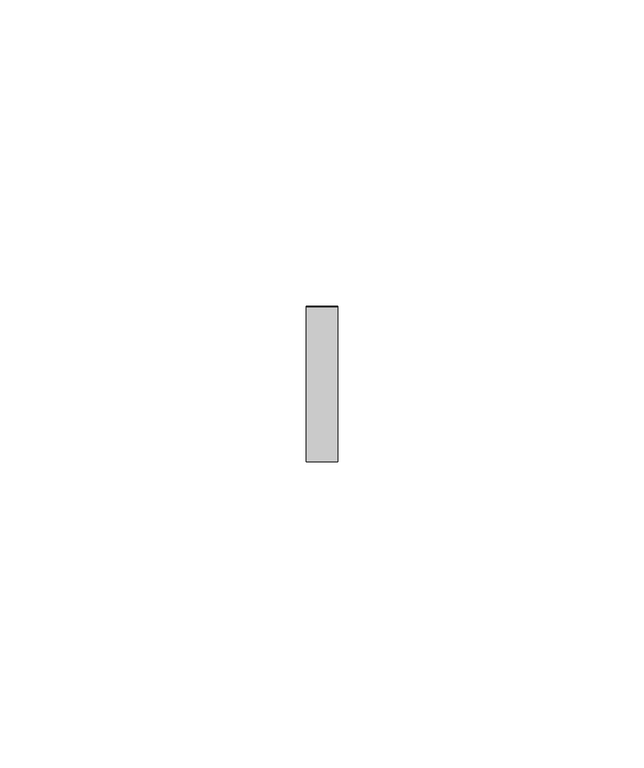
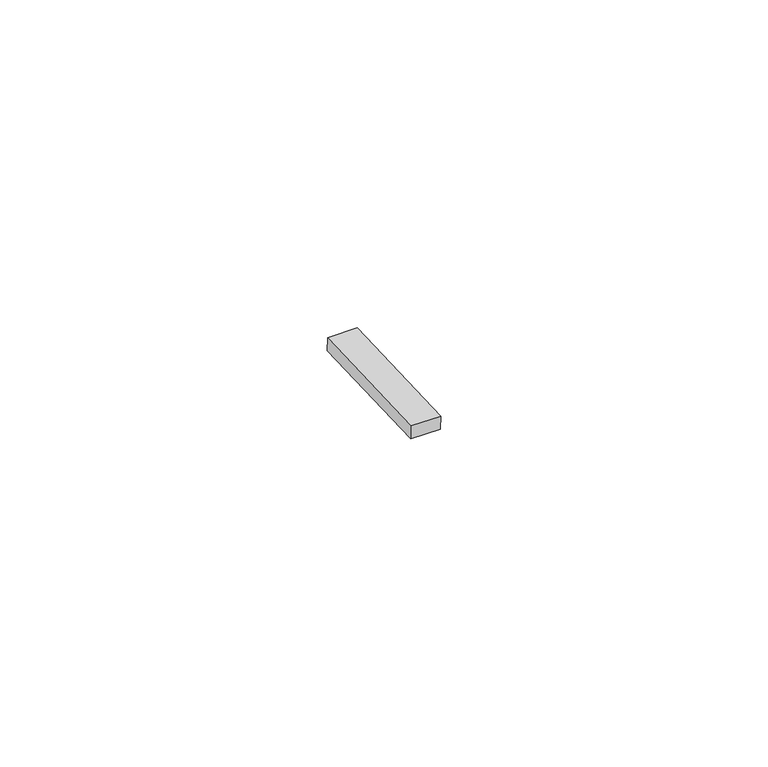
"""IFC4 building model written with IfcOpenShell, lengths in millimetres: proxy geometry, Inner panel:Inner panel:1:Inner panel:1 : Inner panel:Inner panel:300324:2:Inner panel:1:Inner panel:1 : Inner panel:Inner panel:300324:2 : Inner panel:Inner panel:1:Inner panel:1 : Inner panel:Inner panel:300324:300043:134 : Inner panel:Inner panel:1:Inner panel:1 : Inner panel:Inner panel:300324:2:Inner panel:1:Inner panel:1 : Inner panel:Inner panel:300324:2 : Inner panel:Inner panel:1:Inner panel:1 : Inner panel:Inner panel:300324:300043:308120."""

from ifc_helpers import new_model, si_unit, frame, origin, place, context, project, spatial, polyline, outline, extrude, source, transform, mapped, element, save


def generic_models_b44d6d40(model_context):
    return source(origin(), model_context, "Body", "SweptSolid", [
        extrude(outline(polyline([(0.0, -25.3999999), (0.0, 0.0), (5.2138089, 0.0), (5.2138089, -25.3999999), (0.0, -25.3999999)])), frame((593123.795117, -568123.7593241, 8806.3160403), z_axis=(0.0, -0.041630544712223896, 0.9991330730923502), x_axis=(-1.0, 0.0, 0.0)), (0.0, 0.0, 1.0), 2.4763745),
    ])


if __name__ == "__main__":
    model = new_model("IFC4")
    model_context = context("Model", 3, world=origin())
    ifc_project = project(units=[si_unit("LENGTHUNIT", "METRE", prefix="MILLI")], contexts=[model_context])
    site = spatial("IfcSite", under=ifc_project)
    building = spatial("IfcBuilding", under=site)
    placement = place(None, origin())
    generic_models_shape = generic_models_b44d6d40(model_context)
    element("IfcBuildingElementProxy", 1, Name="Inner panel:Inner panel:1:Inner panel:1 : Inner panel:Inner panel:300324:2:Inner panel:1:Inner panel:1 : Inner panel:Inner panel:300324:2 : Inner panel:Inner panel:1:Inner panel:1 : Inner panel:Inner panel:300324:300043:134 : Inner panel:Inner panel:1:Inner panel:1 : Inner panel:Inner panel:300324:2:Inner panel:1:Inner panel:1 : Inner panel:Inner panel:300324:2 : Inner panel:Inner panel:1:Inner panel:1 : Inner panel:Inner panel:300324:300043:308120", ObjectType="Inner panel:Inner panel:1:Inner panel:1 : Inner panel:Inner panel:300324:2:Inner panel:1:Inner panel:1 : Inner panel:Inner panel:300324:2 : Inner panel:Inner panel:1:Inner panel:1 : Inner panel:Inner panel:300324:300043:134 : Inner panel:Inner panel:1:Inner panel:1 : Inner panel:Inner panel:300324:2:Inner panel:1:Inner panel:1 : Inner panel:Inner panel:300324:2 : Inner panel:Inner panel:1:Inner panel:1 : Inner panel:Inner panel:300324:300043:308120", at=placement, inside=building, context=model_context, shape_type="MappedRepresentation", body=[
        mapped(generic_models_shape, transform((0.0, 0.0, 0.0), x_axis=(1.0, 0.0, 0.0), y_axis=(0.0, 1.0, 0.0), z_axis=(0.0, 0.0, 1.0))),
    ])
    save(model, "model.ifc")

# Revit data of these elements
# Type "Inner panel:Inner panel:1:Inner panel:1 : Inner panel:Inner panel:300324:2:Inner panel:1:Inner panel:1 : Inner panel:Inner panel:300324:2 : Inner panel:Inner panel:1:Inner panel:1 : Inner panel:Inner panel:300324:300043:134 : Inner panel:Inner panel:1:Inner panel:1 : Inner panel:Inner panel:300324:2:Inner panel:1:Inner panel:1 : Inner panel:Inner panel:300324:2 : Inner panel:Inner panel:1:Inner panel:1 : Inner panel:Inner panel:300324:300043:308120"
#   NameOverride = "Inner panel:Inner panel:1:Inner panel:1 : Inner panel:Inner panel:300324:2:Inner panel:1:Inner panel:1 : Inner panel:Inner panel:300324:2 : Inner panel:Inner panel:1:Inner panel:1 : Inner panel:Inner panel:300324:300043:308120"
#   ObjectTypeOverride = "Inner panel:1:Inner panel:1 : Inner panel:Inner panel:300324:2 : Inner panel:Inner panel:1:Inner panel:1 : Inner panel:Inner panel:300324:300043"
#   Reference = "Inner panel"
#   Tag = "308120"
# Element 1 (IfcBuildingElementProxy, "Inner panel:Inner panel:1:Inner panel:1 : Inner panel:Inner panel:300324:2:Inner panel:1:Inner panel:1 : Inner panel:Inner panel:300324:2 : Inner panel:Inner panel:1:Inner panel:1 : Inner panel:Inner panel:300324:300043:134 : Inner panel:Inner panel:1:Inner panel:1 : Inner panel:Inner panel:300324:2:Inner panel:1:Inner panel:1 : Inner panel:Inner panel:300324:2 : Inner panel:Inner panel:1:Inner panel:1 : Inner panel:Inner panel:300324:300043:308120")
#   Materials on its faces: "AT CLIP - 1\" WIDE NON ABSORBENT, WEATHER-RESISTANT NEOPRENE/EPDM/SBR FOAM"
# Materials
#   "AT CLIP - 1\" WIDE NON ABSORBENT, WEATHER-RESISTANT NEOPRENE/EPDM/SBR FOAM": class "Generic", colour RGB 85 85 85, transparency 0, Cost = 0
